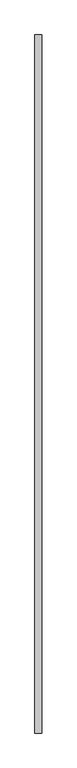
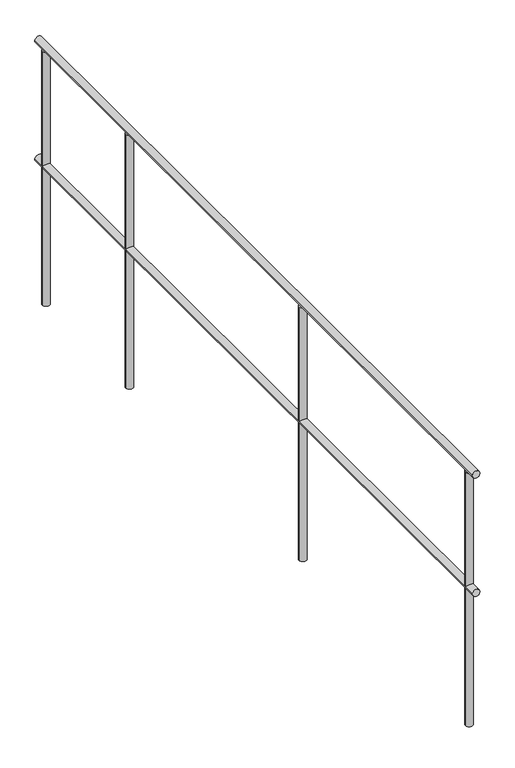
"""IFC4 building model written with IfcOpenShell, lengths in millimetres: railing geometry."""

from ifc_helpers import new_model, si_unit, point, frame, frame_2d, origin, place, context, project, spatial, circle_curve, trimmed, segment, composite_curve, outline, extrude, source, transform, mapped, element, save


def railing_7a6e51f3(model_context):
    return source(origin(), model_context, "Body", "SweptSolid", [
        extrude(outline(composite_curve([segment(trimmed(circle_curve(frame_2d((885.0, 3950.7243044)), 15.0), [point((885.0, 3965.7243044))], [point((885.0, 3935.7243044))], False, "CARTESIAN"), True, "CONTINUOUS"), segment(trimmed(circle_curve(frame_2d((885.0, 3950.7243044)), 15.0), [point((885.0, 3935.7243044))], [point((885.0, 3965.7243044))], False, "CARTESIAN"), True, "CONTINUOUS")], self_intersect=False)), frame((0.0, 60949.5208589, 0.0), z_axis=(0.0, 1.0, 0.0), x_axis=(0.0, 0.0, 1.0)), (0.0, 0.0, 1.0), 3027.5),
        extrude(outline(composite_curve([segment(trimmed(circle_curve(frame_2d((1385.0, 3950.7243044)), 15.0), [point((1385.0, 3965.7243044))], [point((1385.0, 3935.7243044))], False, "CARTESIAN"), True, "CONTINUOUS"), segment(trimmed(circle_curve(frame_2d((1385.0, 3950.7243044)), 15.0), [point((1385.0, 3935.7243044))], [point((1385.0, 3965.7243044))], False, "CARTESIAN"), True, "CONTINUOUS")], self_intersect=False)), frame((0.0, 60949.5208589, 0.0), z_axis=(0.0, 1.0, 0.0), x_axis=(0.0, 0.0, 1.0)), (0.0, 0.0, 1.0), 3027.5),
        extrude(outline(composite_curve([segment(trimmed(circle_curve(frame_2d((3950.7243044, 63349.5208589)), 15.0), [point((3965.7243044, 63349.5208589))], [point((3935.7243044, 63349.5208589))], False, "CARTESIAN"), True, "CONTINUOUS"), segment(trimmed(circle_curve(frame_2d((3950.7243044, 63349.5208589)), 15.0), [point((3935.7243044, 63349.5208589))], [point((3965.7243044, 63349.5208589))], False, "CARTESIAN"), True, "CONTINUOUS")], self_intersect=False)), frame((0.0, 0.0, 300.0), z_axis=(0.0, 0.0, 1.0), x_axis=(1.0, 0.0, 0.0)), (0.0, 0.0, 1.0), 1070.0),
        extrude(outline(composite_curve([segment(trimmed(circle_curve(frame_2d((3950.7243044, 62149.5208589)), 15.0), [point((3965.7243044, 62149.5208589))], [point((3935.7243044, 62149.5208589))], False, "CARTESIAN"), True, "CONTINUOUS"), segment(trimmed(circle_curve(frame_2d((3950.7243044, 62149.5208589)), 15.0), [point((3935.7243044, 62149.5208589))], [point((3965.7243044, 62149.5208589))], False, "CARTESIAN"), True, "CONTINUOUS")], self_intersect=False)), frame((0.0, 0.0, 300.0), z_axis=(0.0, 0.0, 1.0), x_axis=(1.0, 0.0, 0.0)), (0.0, 0.0, 1.0), 1070.0),
        extrude(outline(composite_curve([segment(trimmed(circle_curve(frame_2d((3950.7243044, 63927.0208589)), 15.0), [point((3965.7243044, 63927.0208589))], [point((3935.7243044, 63927.0208589))], False, "CARTESIAN"), True, "CONTINUOUS"), segment(trimmed(circle_curve(frame_2d((3950.7243044, 63927.0208589)), 15.0), [point((3935.7243044, 63927.0208589))], [point((3965.7243044, 63927.0208589))], False, "CARTESIAN"), True, "CONTINUOUS")], self_intersect=False)), frame((0.0, 0.0, 300.0), z_axis=(0.0, 0.0, 1.0), x_axis=(1.0, 0.0, 0.0)), (0.0, 0.0, 1.0), 1070.0),
        extrude(outline(composite_curve([segment(trimmed(circle_curve(frame_2d((3950.7243044, 60999.5208589)), 15.0), [point((3965.7243044, 60999.5208589))], [point((3935.7243044, 60999.5208589))], False, "CARTESIAN"), True, "CONTINUOUS"), segment(trimmed(circle_curve(frame_2d((3950.7243044, 60999.5208589)), 15.0), [point((3935.7243044, 60999.5208589))], [point((3965.7243044, 60999.5208589))], False, "CARTESIAN"), True, "CONTINUOUS")], self_intersect=False)), frame((0.0, 0.0, 300.0), z_axis=(0.0, 0.0, 1.0), x_axis=(1.0, 0.0, 0.0)), (0.0, 0.0, 1.0), 1070.0),
    ])


if __name__ == "__main__":
    model = new_model("IFC4")
    model_context = context("Model", 3, world=origin())
    ifc_project = project(units=[si_unit("LENGTHUNIT", "METRE", prefix="MILLI")], contexts=[model_context])
    site = spatial("IfcSite", under=ifc_project)
    building = spatial("IfcBuilding", under=site)
    placement = place(None, origin())
    railing_shape = railing_7a6e51f3(model_context)
    element("IfcRailing", 1, at=placement, inside=building, context=model_context, shape_type="MappedRepresentation", body=[
        mapped(railing_shape, transform((0.0, 0.0, 0.0), x_axis=(1.0, 0.0, 0.0), y_axis=(0.0, 1.0, 0.0), z_axis=(0.0, 0.0, 1.0))),
    ])
    save(model, "model.ifc")
